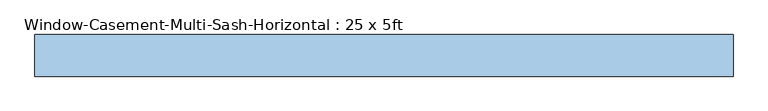
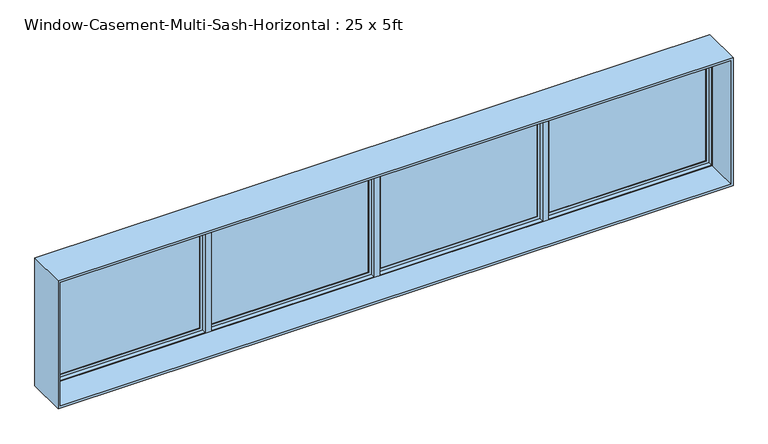
"""IFC4 building model written with IfcOpenShell, lengths in millimetres: window geometry, Window-Casement-Multi-Sash-Horizontal : 25 x 5ft."""

import ifcopenshell
import ifcopenshell.guid

model = None  # the IFC model being written
_history = None  # IfcOwnerHistory: only IFC2X3 demands one
_inside = {}  # id of a spatial element -> (the spatial element, [elements in it])
_under = {}  # id of a project, library or spatial element -> (it, [spatial elements below it])
_declared = {}  # id of a project -> (the project, [libraries it declares])
_typed = {}  # id of a type object -> (the type object, [elements of that type])
_made_of = {}  # id of a material, layer set ... -> (it, [elements and type objects made of it])


def new_model(schema):
    """Start an empty IFC model of exactly this schema.

    Asked for "IFC4X3", IfcOpenShell would pick the latest addendum, in which some entities
    have other attributes; the version numbers below select the first issue.
    IFC2X3 requires an IfcOwnerHistory on every rooted entity: one is made here for all.
    """
    global model, _history
    if schema == "IFC4X3":
        model = ifcopenshell.file(schema_version=(4, 3, 0, 0))
    else:
        model = ifcopenshell.file(schema=schema)
    _inside.clear()
    _under.clear()
    _declared.clear()
    _typed.clear()
    _made_of.clear()
    _history = None
    if model.schema == "IFC2X3":
        org = make("IfcOrganization", Name="unknown")
        user = make(
            "IfcPersonAndOrganization",
            ThePerson=make("IfcPerson", FamilyName="unknown"),
            TheOrganization=org,
        )
        app = make(
            "IfcApplication",
            ApplicationDeveloper=org,
            Version="unknown",
            ApplicationFullName="unknown",
            ApplicationIdentifier="unknown",
        )
        _history = make(
            "IfcOwnerHistory",
            OwningUser=user,
            OwningApplication=app,
            ChangeAction="ADDED",
            CreationDate=0,
        )
    return model


def make(cls, **values):
    """One entity of the class cls with the attributes given. An attribute that is None is left unset."""
    return model.create_entity(
        cls, **{name: value for name, value in values.items() if value is not None}
    )


def rooted(cls, **values):
    """An entity with a GlobalId (a new one), such as an element, a storey or a relation."""
    return make(cls, GlobalId=ifcopenshell.guid.new(), OwnerHistory=_history, **values)


def si_unit(unit_type, name, prefix=None):
    """IfcSIUnit, for example si_unit("LENGTHUNIT", "METRE", prefix="MILLI")."""
    return make("IfcSIUnit", UnitType=unit_type, Prefix=prefix, Name=name)


def assignment(units):
    """IfcUnitAssignment: the units of a project."""
    return None if units is None else make("IfcUnitAssignment", Units=units)


def point(xyz):
    """IfcCartesianPoint."""
    return None if xyz is None else make("IfcCartesianPoint", Coordinates=xyz)


def direction(xyz):
    """IfcDirection."""
    return None if xyz is None else make("IfcDirection", DirectionRatios=xyz)


def frame(location, z_axis=None, x_axis=None):
    """IfcAxis2Placement3D, a coordinate frame: its origin and axes. An axis left out is left unset."""
    return make(
        "IfcAxis2Placement3D",
        Location=point(location),
        Axis=direction(z_axis),
        RefDirection=direction(x_axis),
    )


def origin():
    """The frame at (0, 0, 0) with its axes left unset."""
    return frame((0.0, 0.0, 0.0))


def place(relative_to, where):
    """IfcLocalPlacement: puts the frame where relative to a parent placement (None: the world)."""
    return make(
        "IfcLocalPlacement", PlacementRelTo=relative_to, RelativePlacement=where
    )


def context(
    kind, dimensions, precision=None, world=None, true_north=None, identifier=None
):
    """IfcGeometricRepresentationContext, for example the 3D "Model" context."""
    return make(
        "IfcGeometricRepresentationContext",
        ContextIdentifier=identifier,
        ContextType=kind,
        CoordinateSpaceDimension=dimensions,
        Precision=precision,
        WorldCoordinateSystem=world,
        TrueNorth=true_north,
    )


def project(units=None, contexts=None):
    """IfcProject with its units and contexts."""
    return rooted(
        "IfcProject",
        Name="project",
        RepresentationContexts=contexts,
        UnitsInContext=assignment(units),
    )


def spatial(cls, under=None, at=None, **own):
    """A site, building, storey or space (cls), placed at a placement, below another one or the project."""
    s = rooted(cls, ObjectPlacement=at, **own)
    if under is not None:
        _under.setdefault(under.id(), (under, []))[1].append(s)
    return s


def polyline(points):
    """IfcPolyline through the points."""
    return make("IfcPolyline", Points=[point(p) for p in points])


def outline(outer, holes=None, kind="AREA"):
    """IfcArbitraryClosedProfileDef: a profile drawn as a closed curve; with holes, ...WithVoids."""
    if holes is None:
        return make("IfcArbitraryClosedProfileDef", ProfileType=kind, OuterCurve=outer)
    return make(
        "IfcArbitraryProfileDefWithVoids",
        ProfileType=kind,
        OuterCurve=outer,
        InnerCurves=holes,
    )


def extrude(swept, where, along, depth):
    """IfcExtrudedAreaSolid: the profile swept, set in the frame where, extruded along a direction by depth."""
    return make(
        "IfcExtrudedAreaSolid",
        SweptArea=swept,
        Position=where,
        ExtrudedDirection=direction(along),
        Depth=depth,
    )


def faces_of(points, faces, orient=None, outer=None):
    """IfcFace entities. A face is a list of loops; a loop is a list of indices into points, from 0.

    orient and outer hold one flag for each loop. By default every Orientation is true, the
    first loop of a face is its IfcFaceOuterBound and the others are IfcFaceBound.
    """
    made = []
    for i, loops in enumerate(faces):
        bounds = []
        for j, loop in enumerate(loops):
            is_outer = j == 0 if outer is None else outer[i][j]
            bounds.append(
                make(
                    "IfcFaceOuterBound" if is_outer else "IfcFaceBound",
                    Bound=make("IfcPolyLoop", Polygon=[points[k] for k in loop]),
                    Orientation=True if orient is None else orient[i][j],
                )
            )
        made.append(make("IfcFace", Bounds=bounds))
    return made


def faceted_brep(points, faces, orient=None, outer=None, voids=None):
    """IfcFacetedBrep: a solid bounded by flat faces; with voids (closed shells), ...WithVoids."""
    shared = [point(p) for p in points]
    hull = make("IfcClosedShell", CfsFaces=faces_of(shared, faces, orient, outer))
    if voids is None:
        return make("IfcFacetedBrep", Outer=hull)
    return make(
        "IfcFacetedBrepWithVoids",
        Outer=hull,
        Voids=[
            make(cls, CfsFaces=faces_of(shared, fs, o, b)) for cls, fs, o, b in voids
        ],
    )


def shape(context_of_items, identifier, shape_type, items):
    """IfcShapeRepresentation: the items that make up one representation, for example the "Body"."""
    return make(
        "IfcShapeRepresentation",
        ContextOfItems=context_of_items,
        RepresentationIdentifier=identifier,
        RepresentationType=shape_type,
        Items=items,
    )


def source(mapping_origin, context_of_items, identifier, shape_type, items):
    """IfcRepresentationMap: a shape defined once, which mapped items show again and again."""
    return make(
        "IfcRepresentationMap",
        MappingOrigin=mapping_origin,
        MappedRepresentation=shape(context_of_items, identifier, shape_type, items),
    )


def transform(
    local_origin,
    x_axis=None,
    y_axis=None,
    z_axis=None,
    scale=None,
    scale2=None,
    scale3=None,
    uniform=True,
):
    """IfcCartesianTransformationOperator3D, or its non-uniform kind. x_axis, y_axis, z_axis: its Axis1, 2, 3."""
    if uniform:
        return make(
            "IfcCartesianTransformationOperator3D",
            Axis1=direction(x_axis),
            Axis2=direction(y_axis),
            LocalOrigin=point(local_origin),
            Scale=scale,
            Axis3=direction(z_axis),
        )
    return make(
        "IfcCartesianTransformationOperator3DnonUniform",
        Axis1=direction(x_axis),
        Axis2=direction(y_axis),
        LocalOrigin=point(local_origin),
        Scale=scale,
        Axis3=direction(z_axis),
        Scale2=scale2,
        Scale3=scale3,
    )


def mapped(mapping_source, mapping_target):
    """IfcMappedItem: shows the shape of a source again, moved by a transform."""
    return make(
        "IfcMappedItem", MappingSource=mapping_source, MappingTarget=mapping_target
    )


def made_of(thing, what):
    """Note that an element or type object is made of a material, layer set ...; save() writes the relation."""
    if what is not None:
        _made_of.setdefault(what.id(), (what, []))[1].append(thing)
    return thing


def element(
    cls,
    number,
    at=None,
    inside=None,
    cuts=None,
    type_object=None,
    material=None,
    context=None,
    identifier="Body",
    shape_type=None,
    held_by="IfcProductDefinitionShape",
    body=None,
    shapes=None,
    **own,
):
    """One element of the class cls, such as IfcWall. Its Tag is "e" and its number.

    at: its placement. inside: the storey or other place that contains it. cuts: it is an
    opening in that element (IfcRelVoidsElement). A single representation is given by context,
    identifier, shape_type and body (its items); several are given by shapes. held_by: the class
    of the entity that holds the representations. save() writes the other relations.
    """
    e = rooted(cls, Tag="e%d" % number, ObjectPlacement=at, **own)
    if body is not None:
        shapes = [shape(context, identifier, shape_type, body)]
    if shapes is not None:
        e.Representation = make(held_by, Representations=shapes)
    if inside is not None:
        _inside.setdefault(inside.id(), (inside, []))[1].append(e)
    if cuts is not None:
        rooted(
            "IfcRelVoidsElement", RelatingBuildingElement=cuts, RelatedOpeningElement=e
        )
    if type_object is not None:
        _typed.setdefault(type_object.id(), (type_object, []))[1].append(e)
    return made_of(e, material)


def aggregate(whole, parts):
    """IfcRelAggregates: a whole, such as a stair, and the parts it consists of."""
    return rooted("IfcRelAggregates", RelatingObject=whole, RelatedObjects=parts)


def save(model, path):
    """Write the relations noted so far, then the file.

    IfcRelAggregates (storeys below a building ...), IfcRelContainedInSpatialStructure (elements
    in a storey), IfcRelDefinesByType, IfcRelAssociatesMaterial and IfcRelDeclares: one each for
    every whole, place, type object, material and project.
    """
    for whole, parts in _under.values():
        aggregate(whole, parts)
    for where, things in _inside.values():
        rooted(
            "IfcRelContainedInSpatialStructure",
            RelatedElements=things,
            RelatingStructure=where,
        )
    for kind, things in _typed.values():
        rooted("IfcRelDefinesByType", RelatedObjects=things, RelatingType=kind)
    for what, things in _made_of.values():
        rooted("IfcRelAssociatesMaterial", RelatedObjects=things, RelatingMaterial=what)
    for by, libraries in _declared.values():
        rooted("IfcRelDeclares", RelatingContext=by, RelatedDefinitions=libraries)
    model.write(path)


def window_casement_multi_sash_horizontal_25_x_5ft_0e5d08e3(model_context):
    return source(origin(), model_context, "Body", "SolidModel", [
        extrude(outline(polyline([(2413.0, -1879.6), (939.8, -1879.6), (939.8, -25.4), (2413.0, -25.4), (2413.0, -1879.6)]), holes=[polyline([(2371.1296875, -67.2703125), (981.6703125, -67.2703125), (981.6703125, -1837.7296875), (2371.1296875, -1837.7296875), (2371.1296875, -67.2703125)])]), frame((0.0, 185.7375, 0.0), z_axis=(0.0, 1.0, 0.0), x_axis=(0.0, 0.0, 1.0)), (0.0, 0.0, 1.0), 31.75),
        extrude(outline(polyline([(2413.0, 25.4), (939.8, 25.4), (939.8, 1879.6), (2413.0, 1879.6), (2413.0, 25.4)]), holes=[polyline([(2371.1296875, 1837.7296875), (981.6703125, 1837.7296875), (981.6703125, 67.2703125), (2371.1296875, 67.2703125), (2371.1296875, 1837.7296875)])]), frame((0.0, 185.7375, 0.0), z_axis=(0.0, 1.0, 0.0), x_axis=(0.0, 0.0, 1.0)), (0.0, 0.0, 1.0), 31.75),
        faceted_brep([(-1930.4, 185.7375, 2413.0), (-3784.6, 185.7375, 2413.0), (-3784.6, 227.0125, 2413.0), (3784.6, 227.0125, 2413.0), (3784.6, 185.7375, 2413.0), (1930.4, 185.7375, 2413.0), (1930.4, 223.8375, 2413.0), (1879.6, 223.8375, 2413.0), (1879.6, 185.7375, 2413.0), (25.4, 185.7375, 2413.0), (25.4, 223.8375, 2413.0), (-25.4, 223.8375, 2413.0), (-25.4, 185.7375, 2413.0), (-1879.6, 185.7375, 2413.0), (-1879.6, 223.8375, 2413.0), (-1930.4, 223.8375, 2413.0), (-3774.4796875, 134.9375, 2402.8796875), (-3774.4796875, 185.7375, 2402.8796875), (-1940.5203125, 185.7375, 2402.8796875), (-1940.5203125, 134.9375, 2402.8796875), (3774.4796875, 185.7375, 2402.8796875), (3774.4796875, 134.9375, 2402.8796875), (1940.5203125, 134.9375, 2402.8796875), (1940.5203125, 185.7375, 2402.8796875), (-1869.4796875, 185.7375, 2402.8796875), (-35.5203125, 185.7375, 2402.8796875), (-35.5203125, 134.9375, 2402.8796875), (-1869.4796875, 134.9375, 2402.8796875), (35.5203125, 185.7375, 2402.8796875), (1869.4796875, 185.7375, 2402.8796875), (1869.4796875, 134.9375, 2402.8796875), (35.5203125, 134.9375, 2402.8796875), (-3784.6, -227.0125, 2413.0), (-3784.6, 134.9375, 2413.0), (3784.6, 134.9375, 2413.0), (3784.6, -227.0125, 2413.0), (-3810.0, 227.0125, 2438.4), (-3810.0, -227.0125, 2438.4), (3810.0, -227.0125, 2438.4), (3810.0, 227.0125, 2438.4), (3784.6, 227.0125, 939.8), (3784.6, 185.7375, 939.8), (3774.4796875, 185.7375, 949.9203125), (3774.4796875, 134.9375, 949.9203125), (3784.6, 134.9375, 939.8), (3784.6, -227.0125, 939.8), (3810.0, -227.0125, 914.4), (3810.0, 227.0125, 914.4), (1930.4, 185.7375, 939.8), (-3784.6, 227.0125, 939.8), (-3784.6, 185.7375, 939.8), (-1930.4, 185.7375, 939.8), (-1930.4, 223.8375, 939.8), (-1879.6, 223.8375, 939.8), (-1879.6, 185.7375, 939.8), (-25.4, 185.7375, 939.8), (-25.4, 223.8375, 939.8), (25.4, 223.8375, 939.8), (25.4, 185.7375, 939.8), (1879.6, 185.7375, 939.8), (1879.6, 223.8375, 939.8), (1930.4, 223.8375, 939.8), (1940.5203125, 185.7375, 949.9203125), (1940.5203125, 134.9375, 949.9203125), (-3774.4796875, 185.7375, 949.9203125), (-3774.4796875, 134.9375, 949.9203125), (-1940.5203125, 134.9375, 949.9203125), (-1940.5203125, 185.7375, 949.9203125), (-35.5203125, 185.7375, 949.9203125), (-1869.4796875, 185.7375, 949.9203125), (-1869.4796875, 134.9375, 949.9203125), (-35.5203125, 134.9375, 949.9203125), (1869.4796875, 185.7375, 949.9203125), (35.5203125, 185.7375, 949.9203125), (35.5203125, 134.9375, 949.9203125), (1869.4796875, 134.9375, 949.9203125), (-3784.6, 134.9375, 939.8), (-3784.6, -227.0125, 939.8), (-3810.0, -227.0125, 914.4), (-3810.0, 227.0125, 914.4)], [[[0, 1, 2, 3, 4, 5, 6, 7, 8, 9, 10, 11, 12, 13, 14, 15]], [[16, 17, 18, 19]], [[20, 21, 22, 23]], [[24, 25, 26, 27]], [[28, 29, 30, 31]], [[32, 33, 34, 35]], [[36, 37, 38, 39]], [[4, 3, 40, 41]], [[21, 20, 42, 43]], [[35, 34, 44, 45]], [[39, 38, 46, 47]], [[48, 41, 40, 49, 50, 51, 52, 53, 54, 55, 56, 57, 58, 59, 60, 61]], [[43, 42, 62, 63]], [[64, 65, 66, 67]], [[68, 69, 70, 71]], [[72, 73, 74, 75]], [[45, 44, 76, 77]], [[47, 46, 78, 79]], [[2, 1, 50, 49]], [[4, 41, 48, 5], [20, 23, 62, 42]], [[50, 1, 0, 51], [64, 67, 18, 17]], [[12, 55, 54, 13], [69, 68, 25, 24]], [[8, 59, 58, 9], [73, 72, 29, 28]], [[17, 16, 65, 64]], [[44, 34, 33, 76], [16, 19, 66, 65], [27, 26, 71, 70], [31, 30, 75, 74], [21, 43, 63, 22]], [[33, 32, 77, 76]], [[38, 37, 78, 46], [32, 35, 45, 77]], [[37, 36, 79, 78]], [[36, 39, 47, 79], [3, 2, 49, 40]], [[18, 67, 66, 19]], [[69, 24, 27, 70]], [[53, 14, 13, 54]], [[14, 53, 52, 15]], [[15, 52, 51, 0]], [[25, 68, 71, 26]], [[73, 28, 31, 74]], [[57, 10, 9, 58]], [[10, 57, 56, 11]], [[11, 56, 55, 12]], [[6, 61, 60, 7]], [[7, 60, 59, 8]], [[29, 72, 75, 30]], [[62, 23, 22, 63]], [[61, 6, 5, 48]]]),
        extrude(outline(polyline([(-67.2703125, 211.1375), (-67.2703125, 204.7875), (-1837.7296875, 204.7875), (-1837.7296875, 211.1375), (-67.2703125, 211.1375)])), frame((0.0, 0.0, 981.6703125), z_axis=(0.0, 0.0, 1.0), x_axis=(1.0, 0.0, 0.0)), (0.0, 0.0, 1.0), 1389.459375),
        extrude(outline(polyline([(-67.2703125, 198.4375), (-67.2703125, 192.0875), (-1837.7296875, 192.0875), (-1837.7296875, 198.4375), (-67.2703125, 198.4375)])), frame((0.0, 0.0, 981.6703125), z_axis=(0.0, 0.0, 1.0), x_axis=(1.0, 0.0, 0.0)), (0.0, 0.0, 1.0), 1389.459375),
        extrude(outline(polyline([(1837.7296875, 211.1375), (1837.7296875, 204.7875), (67.2703125, 204.7875), (67.2703125, 211.1375), (1837.7296875, 211.1375)])), frame((0.0, 0.0, 981.6703125), z_axis=(0.0, 0.0, 1.0), x_axis=(1.0, 0.0, 0.0)), (0.0, 0.0, 1.0), 1389.459375),
        extrude(outline(polyline([(1837.7296875, 198.4375), (1837.7296875, 192.0875), (67.2703125, 192.0875), (67.2703125, 198.4375), (1837.7296875, 198.4375)])), frame((0.0, 0.0, 981.6703125), z_axis=(0.0, 0.0, 1.0), x_axis=(1.0, 0.0, 0.0)), (0.0, 0.0, 1.0), 1389.459375),
        extrude(outline(polyline([(-1972.2703125, 211.1375), (-1972.2703125, 204.7875), (-3742.7296875, 204.7875), (-3742.7296875, 211.1375), (-1972.2703125, 211.1375)])), frame((0.0, 0.0, 981.6703125), z_axis=(0.0, 0.0, 1.0), x_axis=(1.0, 0.0, 0.0)), (0.0, 0.0, 1.0), 1389.459375),
        extrude(outline(polyline([(-1972.2703125, 198.4375), (-1972.2703125, 192.0875), (-3742.7296875, 192.0875), (-3742.7296875, 198.4375), (-1972.2703125, 198.4375)])), frame((0.0, 0.0, 981.6703125), z_axis=(0.0, 0.0, 1.0), x_axis=(1.0, 0.0, 0.0)), (0.0, 0.0, 1.0), 1389.459375),
        extrude(outline(polyline([(3742.7296875, 211.1375), (3742.7296875, 204.7875), (1972.2703125, 204.7875), (1972.2703125, 211.1375), (3742.7296875, 211.1375)])), frame((0.0, 0.0, 981.6703125), z_axis=(0.0, 0.0, 1.0), x_axis=(1.0, 0.0, 0.0)), (0.0, 0.0, 1.0), 1389.459375),
        extrude(outline(polyline([(3742.7296875, 198.4375), (3742.7296875, 192.0875), (1972.2703125, 192.0875), (1972.2703125, 198.4375), (3742.7296875, 198.4375)])), frame((0.0, 0.0, 981.6703125), z_axis=(0.0, 0.0, 1.0), x_axis=(1.0, 0.0, 0.0)), (0.0, 0.0, 1.0), 1389.459375),
        extrude(outline(polyline([(2413.0, -3784.6), (939.8, -3784.6), (939.8, -1930.4), (2413.0, -1930.4), (2413.0, -3784.6)]), holes=[polyline([(2371.1296875, -1972.2703125), (981.6703125, -1972.2703125), (981.6703125, -3742.7296875), (2371.1296875, -3742.7296875), (2371.1296875, -1972.2703125)])]), frame((0.0, 185.7375, 0.0), z_axis=(0.0, 1.0, 0.0), x_axis=(0.0, 0.0, 1.0)), (0.0, 0.0, 1.0), 31.75),
        extrude(outline(polyline([(2413.0, 1930.4), (939.8, 1930.4), (939.8, 3784.6), (2413.0, 3784.6), (2413.0, 1930.4)]), holes=[polyline([(2371.1296875, 3742.7296875), (981.6703125, 3742.7296875), (981.6703125, 1972.2703125), (2371.1296875, 1972.2703125), (2371.1296875, 3742.7296875)])]), frame((0.0, 185.7375, 0.0), z_axis=(0.0, 1.0, 0.0), x_axis=(0.0, 0.0, 1.0)), (0.0, 0.0, 1.0), 31.75),
    ])


if __name__ == "__main__":
    model = new_model("IFC4")
    model_context = context("Model", 3, world=origin())
    ifc_project = project(units=[si_unit("LENGTHUNIT", "METRE", prefix="MILLI")], contexts=[model_context])
    site = spatial("IfcSite", under=ifc_project)
    building = spatial("IfcBuilding", under=site)
    placement = place(None, origin())
    window_casement_multi_sash_horizontal_25_x_5ft_shape = window_casement_multi_sash_horizontal_25_x_5ft_0e5d08e3(model_context)
    element("IfcWindow", 1, ObjectType="Window-Casement-Multi-Sash-Horizontal : 25 x 5ft", at=placement, inside=building, context=model_context, shape_type="MappedRepresentation", body=[
        mapped(window_casement_multi_sash_horizontal_25_x_5ft_shape, transform((0.0, 0.0, 0.0), x_axis=(1.0, 0.0, 0.0), y_axis=(0.0, 1.0, 0.0), z_axis=(0.0, 0.0, 1.0))),
    ])
    save(model, "model.ifc")

# Revit data of these elements
# Type "Window-Casement-Multi-Sash-Horizontal : 25 x 5ft"
#   Type Mark = "WT-40"
#   Fire Rating = "0.5h"
#   Assembly Code = "B2020100"
#   Analytic Construction = "Double glazing - domestic"
#   Window Inset [instance default] = 0' - 0 5/8"
#   Wall Thickness [instance default] = 0' - 6"
#   Visual Light Transmittance = 0.81
#   Thermal Resistance (R) = 1.8146 (h·ft²·°F)/BTU
#   Solar Heat Gain Coefficient = 0.76
#   Rough Width = 25' - 0 1/2"
#   Rough Height = 5' - 0 1/2"
#   Open Window Width = 6' - 3"
#   Heat Transfer Coefficient (U) = 0.5511 BTU/(h·ft²·°F)
#   Height = 5' - 0"
#   Frame Gap 3 [instance default] = 0' - 1 83/128"
#   Frame Gap 2 [instance default] = 0' - 0 5/8"
#   Frame Gap 1 = 0' - 1 51/128"
#   Default Sill Height = 3' - 0"
#   Width = 25' - 0"
#   Define Thermal Properties by = 1
#   Frame Material = Metal - Aluminum
#   Glass Panel Material = Glass
#   Wall Closure = (empty or 0)
# Element 1 (IfcWindow, "Window-Casement-Multi-Sash-Horizontal : 25 x 5ft")
#   Wall Thickness = 1' - 5 7/8"
#   Materials on its faces: "Metal - Aluminum", "Glass"
# Materials
#   "Metal - Aluminum": class "Metal", colour RGB 247 247 247, transparency 0
#   "Glass": class "Glass", colour RGB 0 128 192, transparency 0.75, Description = "Soda Lime Glass", Cost = 0
